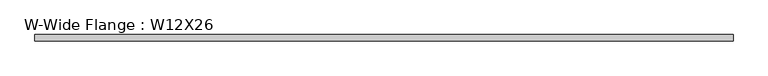
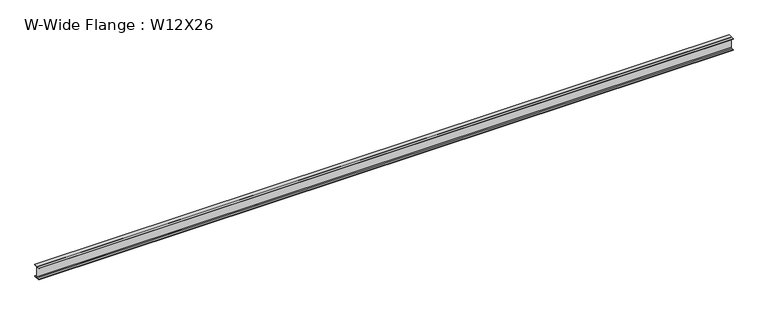
"""IFC4 building model written with IfcOpenShell, lengths in millimetres: beam geometry, W-Wide Flange : W12X26."""

import ifcopenshell
import ifcopenshell.guid

model = None  # the IFC model being written
_history = None  # IfcOwnerHistory: only IFC2X3 demands one
_inside = {}  # id of a spatial element -> (the spatial element, [elements in it])
_under = {}  # id of a project, library or spatial element -> (it, [spatial elements below it])
_declared = {}  # id of a project -> (the project, [libraries it declares])
_typed = {}  # id of a type object -> (the type object, [elements of that type])
_made_of = {}  # id of a material, layer set ... -> (it, [elements and type objects made of it])


def new_model(schema):
    """Start an empty IFC model of exactly this schema.

    Asked for "IFC4X3", IfcOpenShell would pick the latest addendum, in which some entities
    have other attributes; the version numbers below select the first issue.
    IFC2X3 requires an IfcOwnerHistory on every rooted entity: one is made here for all.
    """
    global model, _history
    if schema == "IFC4X3":
        model = ifcopenshell.file(schema_version=(4, 3, 0, 0))
    else:
        model = ifcopenshell.file(schema=schema)
    _inside.clear()
    _under.clear()
    _declared.clear()
    _typed.clear()
    _made_of.clear()
    _history = None
    if model.schema == "IFC2X3":
        org = make("IfcOrganization", Name="unknown")
        user = make(
            "IfcPersonAndOrganization",
            ThePerson=make("IfcPerson", FamilyName="unknown"),
            TheOrganization=org,
        )
        app = make(
            "IfcApplication",
            ApplicationDeveloper=org,
            Version="unknown",
            ApplicationFullName="unknown",
            ApplicationIdentifier="unknown",
        )
        _history = make(
            "IfcOwnerHistory",
            OwningUser=user,
            OwningApplication=app,
            ChangeAction="ADDED",
            CreationDate=0,
        )
    return model


def make(cls, **values):
    """One entity of the class cls with the attributes given. An attribute that is None is left unset."""
    return model.create_entity(
        cls, **{name: value for name, value in values.items() if value is not None}
    )


def rooted(cls, **values):
    """An entity with a GlobalId (a new one), such as an element, a storey or a relation."""
    return make(cls, GlobalId=ifcopenshell.guid.new(), OwnerHistory=_history, **values)


def si_unit(unit_type, name, prefix=None):
    """IfcSIUnit, for example si_unit("LENGTHUNIT", "METRE", prefix="MILLI")."""
    return make("IfcSIUnit", UnitType=unit_type, Prefix=prefix, Name=name)


def assignment(units):
    """IfcUnitAssignment: the units of a project."""
    return None if units is None else make("IfcUnitAssignment", Units=units)


def point(xyz):
    """IfcCartesianPoint."""
    return None if xyz is None else make("IfcCartesianPoint", Coordinates=xyz)


def direction(xyz):
    """IfcDirection."""
    return None if xyz is None else make("IfcDirection", DirectionRatios=xyz)


def frame(location, z_axis=None, x_axis=None):
    """IfcAxis2Placement3D, a coordinate frame: its origin and axes. An axis left out is left unset."""
    return make(
        "IfcAxis2Placement3D",
        Location=point(location),
        Axis=direction(z_axis),
        RefDirection=direction(x_axis),
    )


def frame_2d(location, x_axis=None):
    """IfcAxis2Placement2D, a coordinate frame in the plane: its origin and x axis."""
    return make(
        "IfcAxis2Placement2D", Location=point(location), RefDirection=direction(x_axis)
    )


def origin():
    """The frame at (0, 0, 0) with its axes left unset."""
    return frame((0.0, 0.0, 0.0))


def place(relative_to, where):
    """IfcLocalPlacement: puts the frame where relative to a parent placement (None: the world)."""
    return make(
        "IfcLocalPlacement", PlacementRelTo=relative_to, RelativePlacement=where
    )


def context(
    kind, dimensions, precision=None, world=None, true_north=None, identifier=None
):
    """IfcGeometricRepresentationContext, for example the 3D "Model" context."""
    return make(
        "IfcGeometricRepresentationContext",
        ContextIdentifier=identifier,
        ContextType=kind,
        CoordinateSpaceDimension=dimensions,
        Precision=precision,
        WorldCoordinateSystem=world,
        TrueNorth=true_north,
    )


def project(units=None, contexts=None):
    """IfcProject with its units and contexts."""
    return rooted(
        "IfcProject",
        Name="project",
        RepresentationContexts=contexts,
        UnitsInContext=assignment(units),
    )


def spatial(cls, under=None, at=None, **own):
    """A site, building, storey or space (cls), placed at a placement, below another one or the project."""
    s = rooted(cls, ObjectPlacement=at, **own)
    if under is not None:
        _under.setdefault(under.id(), (under, []))[1].append(s)
    return s


def polyline(points):
    """IfcPolyline through the points."""
    return make("IfcPolyline", Points=[point(p) for p in points])


def circle_curve(where, radius):
    """IfcCircle in the frame where."""
    return make("IfcCircle", Position=where, Radius=radius)


def trimmed(basis, trim1, trim2, sense, master):
    """IfcTrimmedCurve: the piece of a basis curve between two trims."""
    return make(
        "IfcTrimmedCurve",
        BasisCurve=basis,
        Trim1=trim1,
        Trim2=trim2,
        SenseAgreement=sense,
        MasterRepresentation=master,
    )


def segment(curve, same_sense, transition):
    """IfcCompositeCurveSegment."""
    return make(
        "IfcCompositeCurveSegment",
        Transition=transition,
        SameSense=same_sense,
        ParentCurve=curve,
    )


def composite_curve(segments, self_intersect=None):
    """IfcCompositeCurve: segments joined end to end."""
    return make("IfcCompositeCurve", Segments=segments, SelfIntersect=self_intersect)


def outline(outer, holes=None, kind="AREA"):
    """IfcArbitraryClosedProfileDef: a profile drawn as a closed curve; with holes, ...WithVoids."""
    if holes is None:
        return make("IfcArbitraryClosedProfileDef", ProfileType=kind, OuterCurve=outer)
    return make(
        "IfcArbitraryProfileDefWithVoids",
        ProfileType=kind,
        OuterCurve=outer,
        InnerCurves=holes,
    )


def extrude(swept, where, along, depth):
    """IfcExtrudedAreaSolid: the profile swept, set in the frame where, extruded along a direction by depth."""
    return make(
        "IfcExtrudedAreaSolid",
        SweptArea=swept,
        Position=where,
        ExtrudedDirection=direction(along),
        Depth=depth,
    )


def shape(context_of_items, identifier, shape_type, items):
    """IfcShapeRepresentation: the items that make up one representation, for example the "Body"."""
    return make(
        "IfcShapeRepresentation",
        ContextOfItems=context_of_items,
        RepresentationIdentifier=identifier,
        RepresentationType=shape_type,
        Items=items,
    )


def source(mapping_origin, context_of_items, identifier, shape_type, items):
    """IfcRepresentationMap: a shape defined once, which mapped items show again and again."""
    return make(
        "IfcRepresentationMap",
        MappingOrigin=mapping_origin,
        MappedRepresentation=shape(context_of_items, identifier, shape_type, items),
    )


def transform(
    local_origin,
    x_axis=None,
    y_axis=None,
    z_axis=None,
    scale=None,
    scale2=None,
    scale3=None,
    uniform=True,
):
    """IfcCartesianTransformationOperator3D, or its non-uniform kind. x_axis, y_axis, z_axis: its Axis1, 2, 3."""
    if uniform:
        return make(
            "IfcCartesianTransformationOperator3D",
            Axis1=direction(x_axis),
            Axis2=direction(y_axis),
            LocalOrigin=point(local_origin),
            Scale=scale,
            Axis3=direction(z_axis),
        )
    return make(
        "IfcCartesianTransformationOperator3DnonUniform",
        Axis1=direction(x_axis),
        Axis2=direction(y_axis),
        LocalOrigin=point(local_origin),
        Scale=scale,
        Axis3=direction(z_axis),
        Scale2=scale2,
        Scale3=scale3,
    )


def mapped(mapping_source, mapping_target):
    """IfcMappedItem: shows the shape of a source again, moved by a transform."""
    return make(
        "IfcMappedItem", MappingSource=mapping_source, MappingTarget=mapping_target
    )


def made_of(thing, what):
    """Note that an element or type object is made of a material, layer set ...; save() writes the relation."""
    if what is not None:
        _made_of.setdefault(what.id(), (what, []))[1].append(thing)
    return thing


def element(
    cls,
    number,
    at=None,
    inside=None,
    cuts=None,
    type_object=None,
    material=None,
    context=None,
    identifier="Body",
    shape_type=None,
    held_by="IfcProductDefinitionShape",
    body=None,
    shapes=None,
    **own,
):
    """One element of the class cls, such as IfcWall. Its Tag is "e" and its number.

    at: its placement. inside: the storey or other place that contains it. cuts: it is an
    opening in that element (IfcRelVoidsElement). A single representation is given by context,
    identifier, shape_type and body (its items); several are given by shapes. held_by: the class
    of the entity that holds the representations. save() writes the other relations.
    """
    e = rooted(cls, Tag="e%d" % number, ObjectPlacement=at, **own)
    if body is not None:
        shapes = [shape(context, identifier, shape_type, body)]
    if shapes is not None:
        e.Representation = make(held_by, Representations=shapes)
    if inside is not None:
        _inside.setdefault(inside.id(), (inside, []))[1].append(e)
    if cuts is not None:
        rooted(
            "IfcRelVoidsElement", RelatingBuildingElement=cuts, RelatedOpeningElement=e
        )
    if type_object is not None:
        _typed.setdefault(type_object.id(), (type_object, []))[1].append(e)
    return made_of(e, material)


def aggregate(whole, parts):
    """IfcRelAggregates: a whole, such as a stair, and the parts it consists of."""
    return rooted("IfcRelAggregates", RelatingObject=whole, RelatedObjects=parts)


def save(model, path):
    """Write the relations noted so far, then the file.

    IfcRelAggregates (storeys below a building ...), IfcRelContainedInSpatialStructure (elements
    in a storey), IfcRelDefinesByType, IfcRelAssociatesMaterial and IfcRelDeclares: one each for
    every whole, place, type object, material and project.
    """
    for whole, parts in _under.values():
        aggregate(whole, parts)
    for where, things in _inside.values():
        rooted(
            "IfcRelContainedInSpatialStructure",
            RelatedElements=things,
            RelatingStructure=where,
        )
    for kind, things in _typed.values():
        rooted("IfcRelDefinesByType", RelatedObjects=things, RelatingType=kind)
    for what, things in _made_of.values():
        rooted("IfcRelAssociatesMaterial", RelatedObjects=things, RelatingMaterial=what)
    for by, libraries in _declared.values():
        rooted("IfcRelDeclares", RelatingContext=by, RelatedDefinitions=libraries)
    model.write(path)


def w_wide_flange_w12x26_4b0050c2(model_context):
    return source(origin(), model_context, "Body", "SweptSolid", [
        extrude(outline(composite_curve([segment(polyline([(82.4011719, -145.5539063), (82.4011719, -155.178125), (-82.4011719, -155.178125), (-82.4011719, -145.5539063), (-20.2902344, -145.5539063)]), True, "CONTINUOUS"), segment(trimmed(circle_curve(frame_2d((-20.2902344, -128.190625)), 17.3632812), [point((-20.2902344, -145.5539063))], [point((-2.9269531, -128.190625))], True, "CARTESIAN"), True, "CONTINUOUS"), segment(polyline([(-2.9269531, -128.190625), (-2.9269531, 128.190625)]), True, "CONTINUOUS"), segment(trimmed(circle_curve(frame_2d((-20.2902344, 128.190625)), 17.3632812), [point((-2.9269531, 128.190625))], [point((-20.2902344, 145.5539062))], True, "CARTESIAN"), True, "CONTINUOUS"), segment(polyline([(-20.2902344, 145.5539062), (-82.4011719, 145.5539062), (-82.4011719, 155.178125), (82.4011719, 155.178125), (82.4011719, 145.5539062), (20.2902344, 145.5539062)]), True, "CONTINUOUS"), segment(trimmed(circle_curve(frame_2d((20.2902344, 128.190625)), 17.3632812), [point((20.2902344, 145.5539062))], [point((2.9269531, 128.190625))], True, "CARTESIAN"), True, "CONTINUOUS"), segment(polyline([(2.9269531, 128.190625), (2.9269531, -128.190625)]), True, "CONTINUOUS"), segment(trimmed(circle_curve(frame_2d((20.2902344, -128.190625)), 17.3632812), [point((2.9269531, -128.190625))], [point((20.2902344, -145.5539063))], True, "CARTESIAN"), True, "CONTINUOUS"), segment(polyline([(20.2902344, -145.5539063), (82.4011719, -145.5539063)]), True, "CONTINUOUS")], self_intersect=False)), frame((-8743.95, 0.0, 0.0), z_axis=(1.0, 0.0, 0.0), x_axis=(0.0, 1.0, 0.0)), (0.0, 0.0, 1.0), 17487.9),
    ])


if __name__ == "__main__":
    model = new_model("IFC4")
    model_context = context("Model", 3, world=origin())
    ifc_project = project(units=[si_unit("LENGTHUNIT", "METRE", prefix="MILLI")], contexts=[model_context])
    site = spatial("IfcSite", under=ifc_project)
    building = spatial("IfcBuilding", under=site)
    placement = place(None, origin())
    w_wide_flange_w12x26_shape = w_wide_flange_w12x26_4b0050c2(model_context)
    element("IfcBeam", 1, ObjectType="W-Wide Flange : W12X26", at=placement, inside=building, context=model_context, shape_type="MappedRepresentation", body=[
        mapped(w_wide_flange_w12x26_shape, transform((0.0, 0.0, 0.0), x_axis=(1.0, 0.0, 0.0), y_axis=(0.0, 1.0, 0.0), z_axis=(0.0, 0.0, 1.0))),
    ])
    save(model, "model.ifc")

# Revit data of these elements
# Type "W-Wide Flange : W12X26"
#   Assembly Code = "B10"
#   W = 26
#   Length [instance default] = 5' - 0"
#   bf = 0' - 6 125/256"
#   d = 1' - 0 7/32"
#   k = 0' - 1 1/16"
#   k2 = 0' - 0 175/256"
#   tf = 0' - 0 97/256"
#   tw = 0' - 0 59/256"
#   A = 0.053125 SF
#   Structural Material [instance default] = Steel ASTM A992
# Element 1 (IfcBeam, "W-Wide Flange : W12X26")
#   Materials on its faces: "Steel ASTM A992"
# Materials
#   "Steel ASTM A992": class "Metal", colour RGB 199 199 199, transparency 0, Description = "Structural steel 50ksi", Cost = 0
